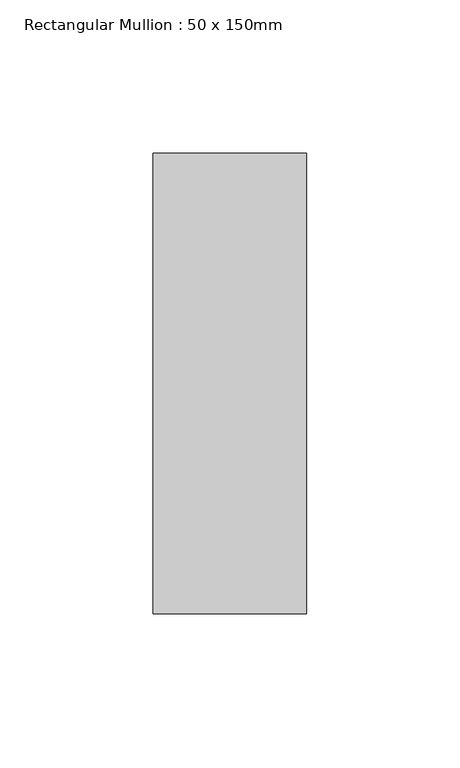
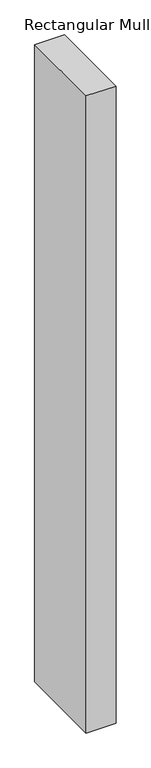
"""IFC4 building model written with IfcOpenShell, lengths in millimetres: member geometry, Rectangular Mullion : 50 x 150mm."""

import ifcopenshell
import ifcopenshell.guid

model = None  # the IFC model being written
_history = None  # IfcOwnerHistory: only IFC2X3 demands one
_inside = {}  # id of a spatial element -> (the spatial element, [elements in it])
_under = {}  # id of a project, library or spatial element -> (it, [spatial elements below it])
_declared = {}  # id of a project -> (the project, [libraries it declares])
_typed = {}  # id of a type object -> (the type object, [elements of that type])
_made_of = {}  # id of a material, layer set ... -> (it, [elements and type objects made of it])


def new_model(schema):
    """Start an empty IFC model of exactly this schema.

    Asked for "IFC4X3", IfcOpenShell would pick the latest addendum, in which some entities
    have other attributes; the version numbers below select the first issue.
    IFC2X3 requires an IfcOwnerHistory on every rooted entity: one is made here for all.
    """
    global model, _history
    if schema == "IFC4X3":
        model = ifcopenshell.file(schema_version=(4, 3, 0, 0))
    else:
        model = ifcopenshell.file(schema=schema)
    _inside.clear()
    _under.clear()
    _declared.clear()
    _typed.clear()
    _made_of.clear()
    _history = None
    if model.schema == "IFC2X3":
        org = make("IfcOrganization", Name="unknown")
        user = make(
            "IfcPersonAndOrganization",
            ThePerson=make("IfcPerson", FamilyName="unknown"),
            TheOrganization=org,
        )
        app = make(
            "IfcApplication",
            ApplicationDeveloper=org,
            Version="unknown",
            ApplicationFullName="unknown",
            ApplicationIdentifier="unknown",
        )
        _history = make(
            "IfcOwnerHistory",
            OwningUser=user,
            OwningApplication=app,
            ChangeAction="ADDED",
            CreationDate=0,
        )
    return model


def make(cls, **values):
    """One entity of the class cls with the attributes given. An attribute that is None is left unset."""
    return model.create_entity(
        cls, **{name: value for name, value in values.items() if value is not None}
    )


def rooted(cls, **values):
    """An entity with a GlobalId (a new one), such as an element, a storey or a relation."""
    return make(cls, GlobalId=ifcopenshell.guid.new(), OwnerHistory=_history, **values)


def si_unit(unit_type, name, prefix=None):
    """IfcSIUnit, for example si_unit("LENGTHUNIT", "METRE", prefix="MILLI")."""
    return make("IfcSIUnit", UnitType=unit_type, Prefix=prefix, Name=name)


def assignment(units):
    """IfcUnitAssignment: the units of a project."""
    return None if units is None else make("IfcUnitAssignment", Units=units)


def point(xyz):
    """IfcCartesianPoint."""
    return None if xyz is None else make("IfcCartesianPoint", Coordinates=xyz)


def direction(xyz):
    """IfcDirection."""
    return None if xyz is None else make("IfcDirection", DirectionRatios=xyz)


def frame(location, z_axis=None, x_axis=None):
    """IfcAxis2Placement3D, a coordinate frame: its origin and axes. An axis left out is left unset."""
    return make(
        "IfcAxis2Placement3D",
        Location=point(location),
        Axis=direction(z_axis),
        RefDirection=direction(x_axis),
    )


def origin():
    """The frame at (0, 0, 0) with its axes left unset."""
    return frame((0.0, 0.0, 0.0))


def place(relative_to, where):
    """IfcLocalPlacement: puts the frame where relative to a parent placement (None: the world)."""
    return make(
        "IfcLocalPlacement", PlacementRelTo=relative_to, RelativePlacement=where
    )


def context(
    kind, dimensions, precision=None, world=None, true_north=None, identifier=None
):
    """IfcGeometricRepresentationContext, for example the 3D "Model" context."""
    return make(
        "IfcGeometricRepresentationContext",
        ContextIdentifier=identifier,
        ContextType=kind,
        CoordinateSpaceDimension=dimensions,
        Precision=precision,
        WorldCoordinateSystem=world,
        TrueNorth=true_north,
    )


def project(units=None, contexts=None):
    """IfcProject with its units and contexts."""
    return rooted(
        "IfcProject",
        Name="project",
        RepresentationContexts=contexts,
        UnitsInContext=assignment(units),
    )


def spatial(cls, under=None, at=None, **own):
    """A site, building, storey or space (cls), placed at a placement, below another one or the project."""
    s = rooted(cls, ObjectPlacement=at, **own)
    if under is not None:
        _under.setdefault(under.id(), (under, []))[1].append(s)
    return s


def polyline(points):
    """IfcPolyline through the points."""
    return make("IfcPolyline", Points=[point(p) for p in points])


def outline(outer, holes=None, kind="AREA"):
    """IfcArbitraryClosedProfileDef: a profile drawn as a closed curve; with holes, ...WithVoids."""
    if holes is None:
        return make("IfcArbitraryClosedProfileDef", ProfileType=kind, OuterCurve=outer)
    return make(
        "IfcArbitraryProfileDefWithVoids",
        ProfileType=kind,
        OuterCurve=outer,
        InnerCurves=holes,
    )


def extrude(swept, where, along, depth):
    """IfcExtrudedAreaSolid: the profile swept, set in the frame where, extruded along a direction by depth."""
    return make(
        "IfcExtrudedAreaSolid",
        SweptArea=swept,
        Position=where,
        ExtrudedDirection=direction(along),
        Depth=depth,
    )


def shape(context_of_items, identifier, shape_type, items):
    """IfcShapeRepresentation: the items that make up one representation, for example the "Body"."""
    return make(
        "IfcShapeRepresentation",
        ContextOfItems=context_of_items,
        RepresentationIdentifier=identifier,
        RepresentationType=shape_type,
        Items=items,
    )


def source(mapping_origin, context_of_items, identifier, shape_type, items):
    """IfcRepresentationMap: a shape defined once, which mapped items show again and again."""
    return make(
        "IfcRepresentationMap",
        MappingOrigin=mapping_origin,
        MappedRepresentation=shape(context_of_items, identifier, shape_type, items),
    )


def transform(
    local_origin,
    x_axis=None,
    y_axis=None,
    z_axis=None,
    scale=None,
    scale2=None,
    scale3=None,
    uniform=True,
):
    """IfcCartesianTransformationOperator3D, or its non-uniform kind. x_axis, y_axis, z_axis: its Axis1, 2, 3."""
    if uniform:
        return make(
            "IfcCartesianTransformationOperator3D",
            Axis1=direction(x_axis),
            Axis2=direction(y_axis),
            LocalOrigin=point(local_origin),
            Scale=scale,
            Axis3=direction(z_axis),
        )
    return make(
        "IfcCartesianTransformationOperator3DnonUniform",
        Axis1=direction(x_axis),
        Axis2=direction(y_axis),
        LocalOrigin=point(local_origin),
        Scale=scale,
        Axis3=direction(z_axis),
        Scale2=scale2,
        Scale3=scale3,
    )


def mapped(mapping_source, mapping_target):
    """IfcMappedItem: shows the shape of a source again, moved by a transform."""
    return make(
        "IfcMappedItem", MappingSource=mapping_source, MappingTarget=mapping_target
    )


def made_of(thing, what):
    """Note that an element or type object is made of a material, layer set ...; save() writes the relation."""
    if what is not None:
        _made_of.setdefault(what.id(), (what, []))[1].append(thing)
    return thing


def element(
    cls,
    number,
    at=None,
    inside=None,
    cuts=None,
    type_object=None,
    material=None,
    context=None,
    identifier="Body",
    shape_type=None,
    held_by="IfcProductDefinitionShape",
    body=None,
    shapes=None,
    **own,
):
    """One element of the class cls, such as IfcWall. Its Tag is "e" and its number.

    at: its placement. inside: the storey or other place that contains it. cuts: it is an
    opening in that element (IfcRelVoidsElement). A single representation is given by context,
    identifier, shape_type and body (its items); several are given by shapes. held_by: the class
    of the entity that holds the representations. save() writes the other relations.
    """
    e = rooted(cls, Tag="e%d" % number, ObjectPlacement=at, **own)
    if body is not None:
        shapes = [shape(context, identifier, shape_type, body)]
    if shapes is not None:
        e.Representation = make(held_by, Representations=shapes)
    if inside is not None:
        _inside.setdefault(inside.id(), (inside, []))[1].append(e)
    if cuts is not None:
        rooted(
            "IfcRelVoidsElement", RelatingBuildingElement=cuts, RelatedOpeningElement=e
        )
    if type_object is not None:
        _typed.setdefault(type_object.id(), (type_object, []))[1].append(e)
    return made_of(e, material)


def aggregate(whole, parts):
    """IfcRelAggregates: a whole, such as a stair, and the parts it consists of."""
    return rooted("IfcRelAggregates", RelatingObject=whole, RelatedObjects=parts)


def save(model, path):
    """Write the relations noted so far, then the file.

    IfcRelAggregates (storeys below a building ...), IfcRelContainedInSpatialStructure (elements
    in a storey), IfcRelDefinesByType, IfcRelAssociatesMaterial and IfcRelDeclares: one each for
    every whole, place, type object, material and project.
    """
    for whole, parts in _under.values():
        aggregate(whole, parts)
    for where, things in _inside.values():
        rooted(
            "IfcRelContainedInSpatialStructure",
            RelatedElements=things,
            RelatingStructure=where,
        )
    for kind, things in _typed.values():
        rooted("IfcRelDefinesByType", RelatedObjects=things, RelatingType=kind)
    for what, things in _made_of.values():
        rooted("IfcRelAssociatesMaterial", RelatedObjects=things, RelatingMaterial=what)
    for by, libraries in _declared.values():
        rooted("IfcRelDeclares", RelatingContext=by, RelatedDefinitions=libraries)
    model.write(path)


def rectangular_mullion_50_x_150mm_abf53936(model_context):
    return source(origin(), model_context, "Body", "SweptSolid", [
        extrude(outline(polyline([(0.0, 75.0), (0.0, -75.0), (-50.0, -75.0), (-50.0, 75.0), (0.0, 75.0)])), frame((0.0, 0.0, -1133.3333333), z_axis=(0.0, 0.0, 1.0), x_axis=(1.0, 0.0, 0.0)), (0.0, 0.0, 1.0), 1133.3333333),
    ])


if __name__ == "__main__":
    model = new_model("IFC4")
    model_context = context("Model", 3, world=origin())
    ifc_project = project(units=[si_unit("LENGTHUNIT", "METRE", prefix="MILLI")], contexts=[model_context])
    site = spatial("IfcSite", under=ifc_project)
    building = spatial("IfcBuilding", under=site)
    placement = place(None, origin())
    rectangular_mullion_50_x_150mm_shape = rectangular_mullion_50_x_150mm_abf53936(model_context)
    element("IfcMember", 1, ObjectType="Rectangular Mullion : 50 x 150mm", at=placement, inside=building, context=model_context, shape_type="MappedRepresentation", body=[
        mapped(rectangular_mullion_50_x_150mm_shape, transform((0.0, 0.0, 0.0), x_axis=(1.0, 0.0, 0.0), y_axis=(0.0, 1.0, 0.0), z_axis=(0.0, 0.0, 1.0))),
    ])
    save(model, "model.ifc")

# Revit data of these elements
# Type "Rectangular Mullion : 50 x 150mm"
#   built-in parameter 1007304 = 0.492126 (stored number, unit not read)
#   built-in parameter 1007301 = 0.082021 (stored number, unit not read)
#   built-in parameter 1007300 = 0.082021 (stored number, unit not read)
# Element 1 (IfcMember, "Rectangular Mullion : 50 x 150mm")
#   Materials on its faces: "Metal - Aluminium"
# Materials
#   "Metal - Aluminium": class "Metal", colour RGB 247 247 247, transparency 0
